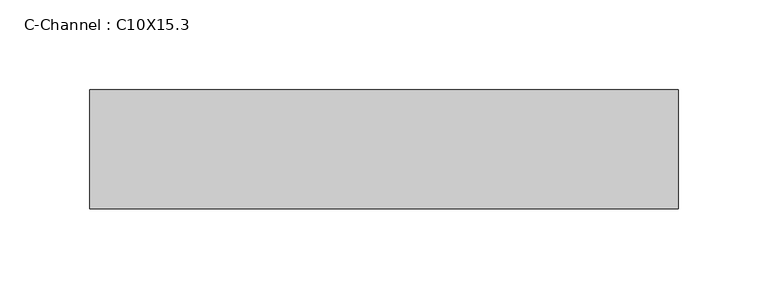
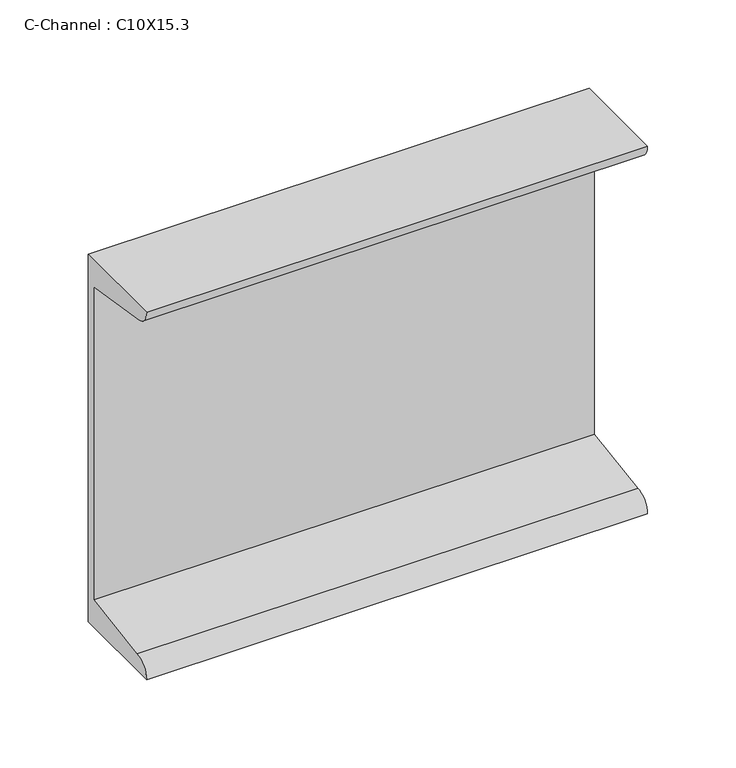
"""IFC4 building model written with IfcOpenShell, lengths in millimetres: beam geometry, C-Channel : C10X15.3."""

from ifc_helpers import new_model, si_unit, point, frame, frame_2d, origin, place, context, project, spatial, polyline, circle_curve, trimmed, segment, composite_curve, outline, extrude, source, transform, mapped, element, save


def c_channel_c10x15_3_182bd023(model_context):
    return source(origin(), model_context, "Body", "SweptSolid", [
        extrude(outline(composite_curve([segment(polyline([(16.1036, 127.0), (16.1036, -127.0), (-49.9364, -127.0)]), True, "CONTINUOUS"), segment(trimmed(circle_curve(frame_2d((-38.862, -127.0)), 11.0744), [point((-49.9364, -127.0))], [point((-38.862, -115.9256))], False, "CARTESIAN"), True, "CONTINUOUS"), segment(polyline([(-38.862, -115.9256), (10.0076, -108.1854158), (10.0076, 108.1854158), (-38.862, 115.9256)]), True, "CONTINUOUS"), segment(trimmed(circle_curve(frame_2d((-38.862, 127.0)), 11.0744), [point((-38.862, 115.9256))], [point((-49.9364, 127.0))], False, "CARTESIAN"), True, "CONTINUOUS"), segment(polyline([(-49.9364, 127.0), (16.1036, 127.0)]), True, "CONTINUOUS")], self_intersect=False)), frame((-124.079, 0.0, 0.0), z_axis=(1.0, 0.0, 0.0), x_axis=(0.0, 1.0, 0.0)), (0.0, 0.0, 1.0), 327.279),
    ])


if __name__ == "__main__":
    model = new_model("IFC4")
    model_context = context("Model", 3, world=origin())
    ifc_project = project(units=[si_unit("LENGTHUNIT", "METRE", prefix="MILLI")], contexts=[model_context])
    site = spatial("IfcSite", under=ifc_project)
    building = spatial("IfcBuilding", under=site)
    placement = place(None, origin())
    c_channel_c10x15_3_shape = c_channel_c10x15_3_182bd023(model_context)
    element("IfcBeam", 1, ObjectType="C-Channel : C10X15.3", at=placement, inside=building, context=model_context, shape_type="MappedRepresentation", body=[
        mapped(c_channel_c10x15_3_shape, transform((0.0, 0.0, 0.0), x_axis=(1.0, 0.0, 0.0), y_axis=(0.0, 1.0, 0.0), z_axis=(0.0, 0.0, 1.0))),
    ])
    save(model, "model.ifc")

# Revit data of these elements
# Type "C-Channel : C10X15.3"
#   Assembly Code = "B10"
#   W = 15.3
#   Length [instance default] = 5' - 0"
#   bf = 0' - 2.6"
#   d = 0' - 10"
#   tf = 0' - 0.436"
#   tw = 0' - 0.24"
#   x = 0' - 0.634"
#   A = 0.0311111 SF
#   Structural Material [instance default] = Steel ASTM A36
# Element 1 (IfcBeam, "C-Channel : C10X15.3")
#   Structural Material = Steel ASTM A992
#   Materials on its faces: "Steel ASTM A992"
# Materials
#   "Steel ASTM A36": class "Metal", colour RGB 199 199 199, transparency 0, Description = "Structural steel, ASTM A36 Grade B, mill finish", Cost = 0
#   "Steel ASTM A992": class "Metal", colour RGB 199 199 199, transparency 0, Description = "Structural steel 50ksi", Cost = 0
